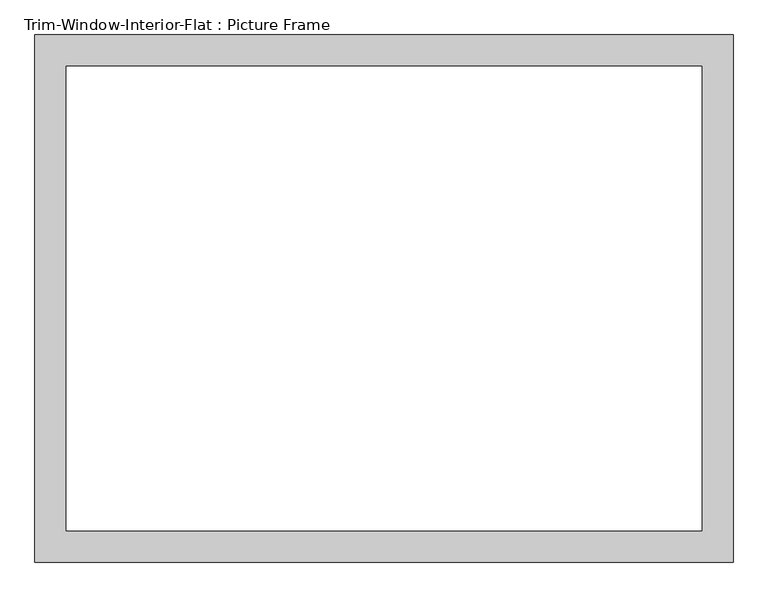
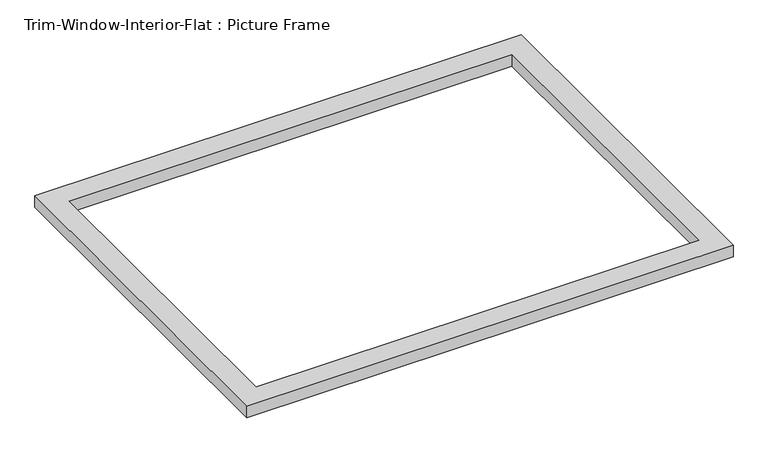
"""IFC4 building model written with IfcOpenShell, lengths in millimetres: proxy geometry, Trim-Window-Interior-Flat : Picture Frame."""

from ifc_helpers import new_model, si_unit, origin, origin_with_axes, place, context, project, spatial, polyline, outline, extrude, source, transform, mapped, element, save


def trim_window_interior_flat_picture_frame_139f52b0(model_context):
    return source(origin(), model_context, "Body", "SweptSolid", [
        extrude(outline(polyline([(635.0, 44.45), (635.0, -914.4), (-635.0, -914.4), (-635.0, 44.45), (635.0, 44.45)]), holes=[polyline([(577.85, -12.7), (-577.85, -12.7), (-577.85, -857.25), (577.85, -857.25), (577.85, -12.7)])]), origin_with_axes(), (0.0, 0.0, 1.0), 31.75),
    ])


if __name__ == "__main__":
    model = new_model("IFC4")
    model_context = context("Model", 3, world=origin())
    ifc_project = project(units=[si_unit("LENGTHUNIT", "METRE", prefix="MILLI")], contexts=[model_context])
    site = spatial("IfcSite", under=ifc_project)
    building = spatial("IfcBuilding", under=site)
    placement = place(None, origin())
    trim_window_interior_flat_picture_frame_shape = trim_window_interior_flat_picture_frame_139f52b0(model_context)
    element("IfcBuildingElementProxy", 1, Name="Trim-Window-Interior-Flat : Picture Frame", ObjectType="Trim-Window-Interior-Flat : Picture Frame", at=placement, inside=building, context=model_context, shape_type="MappedRepresentation", body=[
        mapped(trim_window_interior_flat_picture_frame_shape, transform((0.0, 0.0, 0.0), x_axis=(1.0, 0.0, 0.0), y_axis=(0.0, 1.0, 0.0), z_axis=(0.0, 0.0, 1.0))),
    ])
    save(model, "model.ifc")

# Revit data of these elements
# Type "Trim-Window-Interior-Flat : Picture Frame"
#   Trim Thickness_Picture Frame = 0' - 1 1/4"
#   Trim Width = 0' - 2 1/4"
#   Trim Thickness_with Sill = 0' - 0 3/4"
#   Sill Thickness = 0' - 1 1/4"
#   Opening Width [instance default] = 2' - 0"
#   Opening Height [instance default] = 3' - 0"
#   Default Elevation = 4' - 0"
#   Sill = no
#   Picture Frame = yes
#   Trim Material [instance default] = none
# Element 1 (IfcBuildingElementProxy, "Trim-Window-Interior-Flat : Picture Frame")
#   Opening Width = 3' - 10 1/2"
#   Opening Height = 2' - 10 1/4"
#   Trim Material = Wood - Stained
#   Materials on its faces: "Wood - Stained"
# Materials
#   "Wood - Stained": class "Wood", colour RGB 224 178 126, transparency 0, Cost = 0
